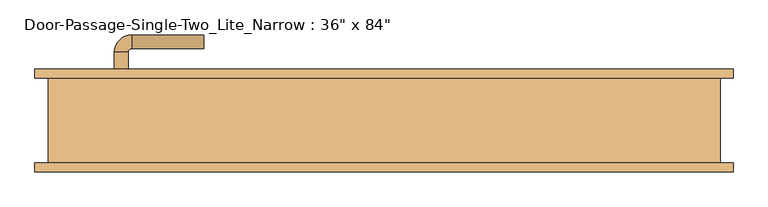
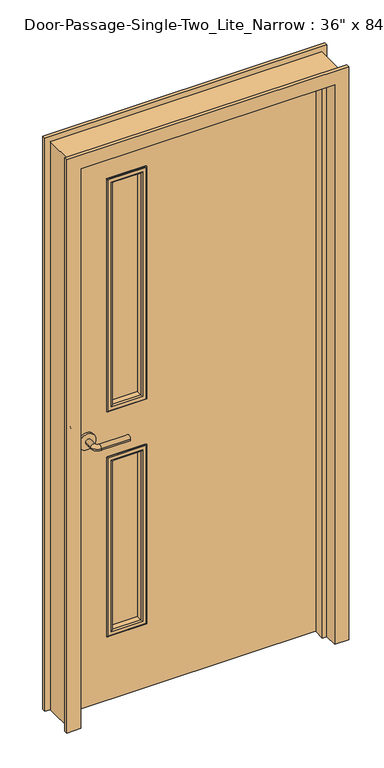
"""IFC4 building model written with IfcOpenShell, lengths in millimetres: door geometry."""

from ifc_helpers import new_model, si_unit, point, frame, frame_2d, origin, place, context, project, spatial, polyline, circle_curve, ellipse_curve, trimmed, segment, composite_curve, outline, extrude, faceted_brep, source, transform, mapped, element, save
from ifc_brep_helpers import plane_surface, cylinder_surface, revolved_surface, advanced_brep


def door_dba893c0(model_context):
    return source(origin(), model_context, "Body", "SolidModel", [
        advanced_brep(
        [(-392.190625, 15.8125, 1016.0), (-372.190625, 15.8125, 1016.0), (-372.190625, -14.1875, 1016.0), (-392.190625, -14.1875, 1016.0), (-367.190625, -19.1875, 1016.0), (-367.190625, -39.1875, 1016.0), (-262.190625, -39.1875, 1016.0), (-262.190625, -19.1875, 1016.0)],
        [
            (0, 1, circle_curve(frame((-382.190625, 15.8125, 1016.0), z_axis=(0.0, 1.0, 0.0), x_axis=(1.0, 0.0, 0.0)), 10.0)),
            (1, 0, circle_curve(frame((-382.190625, 15.8125, 1016.0), z_axis=(0.0, 1.0, 0.0), x_axis=(1.0, 0.0, 0.0)), 10.0)),
            (1, 2),
            (2, 3, circle_curve(frame((-382.190625, -14.1875, 1016.0), z_axis=(0.0, 1.0, 0.0), x_axis=(1.0, 0.0, 0.0)), 10.0)),
            (3, 0),
            (3, 2, circle_curve(frame((-382.190625, -14.1875, 1016.0), z_axis=(0.0, 1.0, 0.0), x_axis=(1.0, 0.0, 0.0)), 10.0)),
            (4, 5, circle_curve(frame((-367.190625, -29.1875, 1016.0), z_axis=(-1.0, 0.0, 0.0), x_axis=(0.0, 1.0, 0.0)), 10.0)),
            (5, 3, circle_curve(frame((-367.190625, -14.1875, 1016.0), z_axis=(0.0, 0.0, -1.0), x_axis=(-1.0, 0.0, 0.0)), 25.0)),
            (2, 4, circle_curve(frame((-367.190625, -14.1875, 1016.0), z_axis=(0.0, 0.0, 1.0), x_axis=(-1.0, 0.0, 0.0)), 5.0)),
            (5, 4, circle_curve(frame((-367.190625, -29.1875, 1016.0), z_axis=(-1.0, 0.0, 0.0), x_axis=(0.0, 1.0, 0.0)), 10.0)),
            (6, 7, circle_curve(frame((-262.190625, -29.1875, 1016.0), z_axis=(1.0, 0.0, 0.0), x_axis=(0.0, 1.0, 0.0)), 10.0)),
            (7, 6, circle_curve(frame((-262.190625, -29.1875, 1016.0), z_axis=(1.0, 0.0, 0.0), x_axis=(0.0, 1.0, 0.0)), 10.0)),
            (4, 7),
            (6, 5),
        ],
        [
            plane_surface(frame((-382.190625, 15.8125, 1016.0), z_axis=(0.0, 1.0, 0.0), x_axis=(0.0, 0.0, 1.0))),
            cylinder_surface(frame((-382.190625, 15.8125, 1016.0), z_axis=(0.0, 1.0, 0.0), x_axis=(1.0, 0.0, 0.0)), 10.0),
            revolved_surface(trimmed(ellipse_curve(frame((-382.190625, -14.1875, 1016.0), z_axis=(0.0, -1.0, 0.0), x_axis=(1.0, 0.0, 0.0)), 10.0, 10.0), [point((-392.190625, -14.1875, 1016.0))], [point((-372.190625, -14.1875, 1016.0))], True, "CARTESIAN"), (-367.190625, -14.1875, 1016.0), (0.0, 0.0, -1.0)),
            revolved_surface(trimmed(ellipse_curve(frame((-382.190625, -14.1875, 1016.0), z_axis=(0.0, -1.0, 0.0), x_axis=(1.0, 0.0, 0.0)), 10.0, 10.0), [point((-372.190625, -14.1875, 1016.0))], [point((-392.190625, -14.1875, 1016.0))], True, "CARTESIAN"), (-367.190625, -14.1875, 1016.0), (0.0, 0.0, -1.0)),
            plane_surface(frame((-262.190625, -29.1875, 1016.0), z_axis=(1.0, 0.0, 0.0), x_axis=(0.0, 0.0, 1.0))),
            cylinder_surface(frame((-367.190625, -29.1875, 1016.0), z_axis=(-1.0, 0.0, 0.0), x_axis=(0.0, 1.0, 0.0)), 10.0),
        ],
        [
            (0, [[1, 2]]),
            (1, [[3, 4, 5, -2]]),
            (1, [[-5, 6, -3, -1]]),
            (2, [[7, 8, -4, 9]]),
            (3, [[10, -9, -6, -8]]),
            (4, [[11, 12]]),
            (5, [[13, -11, 14, -7]]),
            (5, [[-14, -12, -13, -10]]),
        ],
    ),
        extrude(outline(composite_curve([segment(trimmed(circle_curve(frame_2d((1016.0, -384.690625)), 30.0), [point((1016.0, -414.690625))], [point((1016.0, -354.690625))], False, "CARTESIAN"), True, "CONTINUOUS"), segment(trimmed(circle_curve(frame_2d((1016.0, -384.690625)), 30.0), [point((1016.0, -354.690625))], [point((1016.0, -414.690625))], False, "CARTESIAN"), True, "CONTINUOUS")], self_intersect=False)), frame((0.0, 15.8125, 0.0), z_axis=(0.0, 1.0, 0.0), x_axis=(0.0, 0.0, 1.0)), (0.0, 0.0, 1.0), 8.0),
        advanced_brep(
        [(-392.190625, 76.2625, 1016.0), (-372.190625, 76.2625, 1016.0), (-392.190625, 106.2625, 1016.0), (-372.190625, 106.2625, 1016.0), (-367.190625, 111.2625, 1016.0), (-367.190625, 131.2625, 1016.0), (-262.190625, 131.2625, 1016.0), (-262.190625, 111.2625, 1016.0)],
        [
            (0, 1, circle_curve(frame((-382.190625, 76.2625, 1016.0), z_axis=(0.0, -1.0, 0.0), x_axis=(1.0, 0.0, 0.0)), 10.0)),
            (1, 0, circle_curve(frame((-382.190625, 76.2625, 1016.0), z_axis=(0.0, -1.0, 0.0), x_axis=(1.0, 0.0, 0.0)), 10.0)),
            (0, 2),
            (2, 3, circle_curve(frame((-382.190625, 106.2625, 1016.0), z_axis=(0.0, -1.0, 0.0), x_axis=(1.0, 0.0, 0.0)), 10.0)),
            (3, 1),
            (3, 2, circle_curve(frame((-382.190625, 106.2625, 1016.0), z_axis=(0.0, -1.0, 0.0), x_axis=(1.0, 0.0, 0.0)), 10.0)),
            (4, 3, circle_curve(frame((-367.190625, 106.2625, 1016.0), z_axis=(0.0, 0.0, 1.0), x_axis=(-1.0, 0.0, 0.0)), 5.0)),
            (2, 5, circle_curve(frame((-367.190625, 106.2625, 1016.0), z_axis=(0.0, 0.0, -1.0), x_axis=(-1.0, 0.0, 0.0)), 25.0)),
            (5, 4, circle_curve(frame((-367.190625, 121.2625, 1016.0), z_axis=(-1.0, 0.0, 0.0), x_axis=(0.0, -1.0, 0.0)), 10.0)),
            (4, 5, circle_curve(frame((-367.190625, 121.2625, 1016.0), z_axis=(-1.0, 0.0, 0.0), x_axis=(0.0, -1.0, 0.0)), 10.0)),
            (6, 7, circle_curve(frame((-262.190625, 121.2625, 1016.0), z_axis=(1.0, 0.0, 0.0), x_axis=(0.0, -1.0, 0.0)), 10.0)),
            (7, 6, circle_curve(frame((-262.190625, 121.2625, 1016.0), z_axis=(1.0, 0.0, 0.0), x_axis=(0.0, -1.0, 0.0)), 10.0)),
            (5, 6),
            (7, 4),
        ],
        [
            plane_surface(frame((-382.190625, 76.2625, 1016.0), z_axis=(0.0, -1.0, 0.0), x_axis=(0.0, 0.0, 1.0))),
            cylinder_surface(frame((-382.190625, 76.2625, 1016.0), z_axis=(0.0, -1.0, 0.0), x_axis=(1.0, 0.0, 0.0)), 10.0),
            revolved_surface(trimmed(ellipse_curve(frame((-382.190625, 106.2625, 1016.0), z_axis=(0.0, -1.0, 0.0), x_axis=(1.0, 0.0, 0.0)), 10.0, 10.0), [point((-392.190625, 106.2625, 1016.0))], [point((-372.190625, 106.2625, 1016.0))], True, "CARTESIAN"), (-367.190625, 106.2625, 1016.0), (0.0, 0.0, -1.0)),
            revolved_surface(trimmed(ellipse_curve(frame((-382.190625, 106.2625, 1016.0), z_axis=(0.0, -1.0, 0.0), x_axis=(1.0, 0.0, 0.0)), 10.0, 10.0), [point((-372.190625, 106.2625, 1016.0))], [point((-392.190625, 106.2625, 1016.0))], True, "CARTESIAN"), (-367.190625, 106.2625, 1016.0), (0.0, 0.0, -1.0)),
            plane_surface(frame((-262.190625, 121.2625, 1016.0), z_axis=(1.0, 0.0, 0.0), x_axis=(0.0, 0.0, 1.0))),
            cylinder_surface(frame((-367.190625, 121.2625, 1016.0), z_axis=(-1.0, 0.0, 0.0), x_axis=(0.0, -1.0, 0.0)), 10.0),
        ],
        [
            (0, [[1, 2]]),
            (1, [[-1, 3, 4, 5]]),
            (1, [[-2, -5, 6, -3]]),
            (2, [[7, -4, 8, 9]]),
            (3, [[-8, -6, -7, 10]]),
            (4, [[11, 12]]),
            (5, [[-9, 13, -12, 14]]),
            (5, [[-10, -14, -11, -13]]),
        ],
    ),
        extrude(outline(composite_curve([segment(trimmed(circle_curve(frame_2d((1016.0, -384.690625)), 30.0), [point((1016.0, -414.690625))], [point((1016.0, -354.690625))], False, "CARTESIAN"), True, "CONTINUOUS"), segment(trimmed(circle_curve(frame_2d((1016.0, -384.690625)), 30.0), [point((1016.0, -354.690625))], [point((1016.0, -414.690625))], False, "CARTESIAN"), True, "CONTINUOUS")], self_intersect=False)), frame((0.0, 68.2625, 0.0), z_axis=(0.0, 1.0, 0.0), x_axis=(0.0, 0.0, 1.0)), (0.0, 0.0, 1.0), 8.0),
        faceted_brep([(457.2, 80.9625, 0.0), (508.0, 80.9625, 0.0), (508.0, 68.2625, 0.0), (488.95, 68.2625, 0.0), (488.95, -55.5625, 0.0), (508.0, -55.5625, 0.0), (508.0, -68.2625, 0.0), (457.2, -68.2625, 0.0), (457.2, -19.05, 0.0), (441.325, -19.05, 0.0), (441.325, 19.05, 0.0), (457.2, 19.05, 0.0), (457.2, 80.9625, 2133.6), (-457.2, 80.9625, 2133.6), (-457.2, 80.9625, 0.0), (-508.0, 80.9625, 0.0), (-508.0, 80.9625, 2184.4), (508.0, 80.9625, 2184.4), (508.0, 68.2625, 2184.4), (-508.0, 68.2625, 2184.4), (-508.0, 68.2625, 0.0), (-488.95, 68.2625, 0.0), (-488.95, 68.2625, 2165.35), (488.95, 68.2625, 2165.35), (488.95, -55.5625, 2165.35), (-488.95, -55.5625, 2165.35), (-488.95, -55.5625, 0.0), (-508.0, -55.5625, 0.0), (-508.0, -55.5625, 2184.4), (508.0, -55.5625, 2184.4), (508.0, -68.2625, 2184.4), (-508.0, -68.2625, 2184.4), (-508.0, -68.2625, 0.0), (-457.2, -68.2625, 0.0), (-457.2, -68.2625, 2133.6), (457.2, -68.2625, 2133.6), (457.2, -19.05, 2133.6), (-457.2, -19.05, 2133.6), (-457.2, -19.05, 0.0), (-441.325, -19.05, 0.0), (-441.325, -19.05, 2117.725), (441.325, -19.05, 2117.725), (441.325, 19.05, 2117.725), (-441.325, 19.05, 2117.725), (-441.325, 19.05, 0.0), (-457.2, 19.05, 0.0), (-457.2, 19.05, 2133.6), (457.2, 19.05, 2133.6)], [[[0, 1, 2, 3, 4, 5, 6, 7, 8, 9, 10, 11]], [[1, 0, 12, 13, 14, 15, 16, 17]], [[2, 1, 17, 18]], [[3, 2, 18, 19, 20, 21, 22, 23]], [[4, 3, 23, 24]], [[5, 4, 24, 25, 26, 27, 28, 29]], [[6, 5, 29, 30]], [[7, 6, 30, 31, 32, 33, 34, 35]], [[8, 7, 35, 36]], [[9, 8, 36, 37, 38, 39, 40, 41]], [[10, 9, 41, 42]], [[11, 10, 42, 43, 44, 45, 46, 47]], [[0, 11, 47, 12]], [[18, 17, 16, 19]], [[24, 23, 22, 25]], [[30, 29, 28, 31]], [[36, 35, 34, 37]], [[42, 41, 40, 43]], [[12, 47, 46, 13]], [[14, 45, 44, 39, 38, 33, 32, 27, 26, 21, 20, 15]], [[19, 16, 15, 20]], [[25, 22, 21, 26]], [[31, 28, 27, 32]], [[37, 34, 33, 38]], [[43, 40, 39, 44]], [[13, 46, 45, 14]]]),
        extrude(outline(polyline([(2133.6, -457.2), (0.0, -457.2), (0.0, 457.2), (2133.6, 457.2), (2133.6, -457.2)]), holes=[polyline([(1981.2, -304.8), (1981.2, -177.8), (1111.25, -177.8), (1111.25, -304.8), (1981.2, -304.8)]), polyline([(920.75, -304.8), (920.75, -177.8), (254.0, -177.8), (254.0, -304.8), (920.75, -304.8)])]), frame((0.0, 23.8125, 0.0), z_axis=(0.0, 1.0, 0.0), x_axis=(0.0, 0.0, 1.0)), (0.0, 0.0, 1.0), 44.45),
        extrude(outline(polyline([(-177.8, 42.8625), (-304.8, 42.8625), (-304.8, 49.2125), (-177.8, 49.2125), (-177.8, 42.8625)])), frame((0.0, 0.0, 1111.25), z_axis=(0.0, 0.0, 1.0), x_axis=(1.0, 0.0, 0.0)), (0.0, 0.0, 1.0), 869.95),
        extrude(outline(polyline([(-177.8, 42.8625), (-304.8, 42.8625), (-304.8, 49.2125), (-177.8, 49.2125), (-177.8, 42.8625)])), frame((0.0, 0.0, 254.0), z_axis=(0.0, 0.0, 1.0), x_axis=(1.0, 0.0, 0.0)), (0.0, 0.0, 1.0), 666.75),
        advanced_brep(
        [(-177.8, 42.8625, 920.75), (-177.8, 23.8125, 920.75), (-177.8, 23.8125, 254.0), (-177.8, 42.8625, 254.0), (-189.8, 22.8125, 908.75), (-189.8, 42.8625, 908.75), (-189.8, 42.8625, 266.0), (-189.8, 22.8125, 266.0), (-184.8, 17.8125, 913.75), (-184.8, 17.8125, 261.0), (-169.8, 19.8125, 928.75), (-171.8, 17.8125, 926.75), (-171.8, 17.8125, 248.0), (-169.8, 19.8125, 246.0), (-169.8, 23.8125, 928.75), (-169.8, 23.8125, 246.0), (-304.8, 23.8125, 254.0), (-304.8, 42.8625, 254.0), (-292.8, 42.8625, 266.0), (-292.8, 22.8125, 266.0), (-297.8, 17.8125, 261.0), (-310.8, 17.8125, 248.0), (-312.8, 19.8125, 246.0), (-312.8, 23.8125, 246.0), (-304.8, 23.8125, 920.75), (-304.8, 42.8625, 920.75), (-292.8, 42.8625, 908.75), (-292.8, 22.8125, 908.75), (-297.8, 17.8125, 913.75), (-310.8, 17.8125, 926.75), (-312.8, 19.8125, 928.75), (-312.8, 23.8125, 928.75)],
        [
            (0, 1),
            (1, 2),
            (2, 3),
            (3, 0),
            (4, 5),
            (5, 6),
            (6, 7),
            (7, 4),
            (8, 4, ellipse_curve(frame((-184.8, 22.8125, 913.75), z_axis=(0.7071067811865475, 0.0, -0.7071067811865475), x_axis=(0.7071067811865474, 0.0, 0.7071067811865476)), 7.0710678, 5.0)),
            (7, 9, ellipse_curve(frame((-184.8, 22.8125, 261.0), z_axis=(0.7071067811865475, 0.0, 0.7071067811865475), x_axis=(-0.7071067811865474, 0.0, 0.7071067811865476)), 7.0710678, 5.0)),
            (9, 8),
            (10, 11, ellipse_curve(frame((-171.8, 19.8125, 926.75), z_axis=(0.7071067811865475, 0.0, -0.7071067811865475), x_axis=(0.7071067811865474, 0.0, 0.7071067811865476)), 2.8284271, 2.0)),
            (11, 12),
            (12, 13, ellipse_curve(frame((-171.8, 19.8125, 248.0), z_axis=(0.7071067811865475, 0.0, 0.7071067811865475), x_axis=(-0.7071067811865474, 0.0, 0.7071067811865476)), 2.8284271, 2.0)),
            (13, 10),
            (14, 10),
            (13, 15),
            (15, 14),
            (2, 16),
            (16, 17),
            (17, 3),
            (6, 18),
            (18, 19),
            (19, 7),
            (19, 20, ellipse_curve(frame((-297.8, 22.8125, 261.0), z_axis=(0.7071067811865475, 0.0, -0.7071067811865475), x_axis=(0.7071067811865476, 0.0, 0.7071067811865474)), 7.0710678, 5.0)),
            (20, 9),
            (12, 21),
            (21, 22, ellipse_curve(frame((-310.8, 19.8125, 248.0), z_axis=(0.7071067811865475, 0.0, -0.7071067811865475), x_axis=(0.7071067811865476, 0.0, 0.7071067811865474)), 2.8284271, 2.0)),
            (22, 13),
            (22, 23),
            (23, 15),
            (16, 24),
            (24, 25),
            (25, 17),
            (18, 26),
            (26, 27),
            (27, 19),
            (27, 28, ellipse_curve(frame((-297.8, 22.8125, 913.75), z_axis=(-0.7071067811865475, 0.0, -0.7071067811865475), x_axis=(0.7071067811865474, 0.0, -0.7071067811865476)), 7.0710678, 5.0)),
            (28, 20),
            (21, 29),
            (29, 30, ellipse_curve(frame((-310.8, 19.8125, 926.75), z_axis=(-0.7071067811865475, 0.0, -0.7071067811865475), x_axis=(0.7071067811865474, 0.0, -0.7071067811865476)), 2.8284271, 2.0)),
            (30, 22),
            (30, 31),
            (31, 23),
            (31, 14),
            (1, 24),
            (0, 25),
            (5, 26),
            (4, 27),
            (8, 28),
            (11, 29),
            (10, 30),
        ],
        [
            plane_surface(frame((-177.8, 23.8125, 920.75), z_axis=(1.0, 0.0, 0.0), x_axis=(0.0, 0.0, -1.0))),
            plane_surface(frame((-189.8, 42.8625, 908.75), z_axis=(-1.0, 0.0, 0.0), x_axis=(0.0, 0.0, -1.0))),
            cylinder_surface(frame((-184.8, 22.8125, 920.75), z_axis=(0.0, 0.0, 1.0), x_axis=(1.0, 0.0, 0.0)), 5.0),
            cylinder_surface(frame((-171.8, 19.8125, 920.75), z_axis=(0.0, 0.0, 1.0), x_axis=(1.0, 0.0, 0.0)), 2.0),
            plane_surface(frame((-169.8, 19.8125, 928.75), z_axis=(1.0, 0.0, 0.0), x_axis=(0.0, 0.0, -1.0))),
            plane_surface(frame((-177.8, 23.8125, 254.0), z_axis=(0.0, 0.0, -1.0), x_axis=(-1.0, 0.0, 0.0))),
            plane_surface(frame((-189.8, 42.8625, 266.0), z_axis=(0.0, 0.0, 1.0), x_axis=(-1.0, 0.0, 0.0))),
            cylinder_surface(frame((-177.8, 22.8125, 261.0), z_axis=(1.0, 0.0, 0.0), x_axis=(0.0, 0.0, -1.0)), 5.0),
            cylinder_surface(frame((-177.8, 19.8125, 248.0), z_axis=(1.0, 0.0, 0.0), x_axis=(0.0, 0.0, -1.0)), 2.0),
            plane_surface(frame((-169.8, 19.8125, 246.0), z_axis=(0.0, 0.0, -1.0), x_axis=(-1.0, 0.0, 0.0))),
            plane_surface(frame((-304.8, 23.8125, 254.0), z_axis=(-1.0, 0.0, 0.0), x_axis=(0.0, 0.0, 1.0))),
            plane_surface(frame((-292.8, 42.8625, 266.0), z_axis=(1.0, 0.0, 0.0), x_axis=(0.0, 0.0, 1.0))),
            cylinder_surface(frame((-297.8, 22.8125, 254.0), z_axis=(0.0, 0.0, -1.0), x_axis=(-1.0, 0.0, 0.0)), 5.0),
            cylinder_surface(frame((-310.8, 19.8125, 254.0), z_axis=(0.0, 0.0, -1.0), x_axis=(-1.0, 0.0, 0.0)), 2.0),
            plane_surface(frame((-312.8, 19.8125, 246.0), z_axis=(-1.0, 0.0, 0.0), x_axis=(0.0, 0.0, 1.0))),
            plane_surface(frame((-312.8, 23.8125, 928.75), z_axis=(0.0, 1.0, 0.0), x_axis=(1.0, 0.0, 0.0))),
            plane_surface(frame((-304.8, 23.8125, 920.75), z_axis=(0.0, 0.0, 1.0), x_axis=(1.0, 0.0, 0.0))),
            plane_surface(frame((-304.8, 42.8625, 920.75), z_axis=(0.0, 1.0, 0.0), x_axis=(1.0, 0.0, 0.0))),
            plane_surface(frame((-292.8, 42.8625, 908.75), z_axis=(0.0, 0.0, -1.0), x_axis=(1.0, 0.0, 0.0))),
            cylinder_surface(frame((-304.8, 22.8125, 913.75), z_axis=(-1.0, 0.0, 0.0), x_axis=(0.0, 0.0, 1.0)), 5.0),
            plane_surface(frame((-297.8, 17.8125, 913.75), z_axis=(0.0, -1.0, 0.0), x_axis=(1.0, 0.0, 0.0))),
            cylinder_surface(frame((-304.8, 19.8125, 926.75), z_axis=(-1.0, 0.0, 0.0), x_axis=(0.0, 0.0, 1.0)), 2.0),
            plane_surface(frame((-312.8, 19.8125, 928.75), z_axis=(0.0, 0.0, 1.0), x_axis=(1.0, 0.0, 0.0))),
        ],
        [
            (0, [[1, 2, 3, 4]]),
            (1, [[5, 6, 7, 8]]),
            (2, [[9, -8, 10, 11]]),
            (3, [[12, 13, 14, 15]]),
            (4, [[16, -15, 17, 18]]),
            (5, [[-3, 19, 20, 21]]),
            (6, [[-7, 22, 23, 24]]),
            (7, [[-10, -24, 25, 26]]),
            (8, [[-14, 27, 28, 29]]),
            (9, [[-17, -29, 30, 31]]),
            (10, [[-20, 32, 33, 34]]),
            (11, [[-23, 35, 36, 37]]),
            (12, [[-25, -37, 38, 39]]),
            (13, [[-28, 40, 41, 42]]),
            (14, [[-30, -42, 43, 44]]),
            (15, [[-31, -44, 45, -18], [46, -32, -19, -2]]),
            (16, [[-33, -46, -1, 47]]),
            (17, [[-21, -34, -47, -4], [48, -35, -22, -6]]),
            (18, [[-36, -48, -5, 49]]),
            (19, [[-38, -49, -9, 50]]),
            (20, [[51, -40, -27, -13], [-26, -39, -50, -11]]),
            (21, [[-41, -51, -12, 52]]),
            (22, [[-43, -52, -16, -45]]),
        ],
    ),
        advanced_brep(
        [(-304.8, 49.2125, 920.75), (-304.8, 68.2625, 920.75), (-304.8, 68.2625, 254.0), (-304.8, 49.2125, 254.0), (-292.8, 69.2625, 908.75), (-292.8, 49.2125, 908.75), (-292.8, 49.2125, 266.0), (-292.8, 69.2625, 266.0), (-297.8, 74.2625, 913.75), (-297.8, 74.2625, 261.0), (-312.8, 72.2625, 928.75), (-310.8, 74.2625, 926.75), (-310.8, 74.2625, 248.0), (-312.8, 72.2625, 246.0), (-312.8, 68.2625, 928.75), (-312.8, 68.2625, 246.0), (-177.8, 68.2625, 254.0), (-177.8, 49.2125, 254.0), (-189.8, 49.2125, 266.0), (-189.8, 69.2625, 266.0), (-184.8, 74.2625, 261.0), (-171.8, 74.2625, 248.0), (-169.8, 72.2625, 246.0), (-169.8, 68.2625, 246.0), (-177.8, 68.2625, 920.75), (-177.8, 49.2125, 920.75), (-189.8, 49.2125, 908.75), (-189.8, 69.2625, 908.75), (-184.8, 74.2625, 913.75), (-171.8, 74.2625, 926.75), (-169.8, 72.2625, 928.75), (-169.8, 68.2625, 928.75)],
        [
            (0, 1),
            (1, 2),
            (2, 3),
            (3, 0),
            (4, 5),
            (5, 6),
            (6, 7),
            (7, 4),
            (8, 4, ellipse_curve(frame((-297.8, 69.2625, 913.75), z_axis=(-0.7071067811865475, 0.0, -0.7071067811865475), x_axis=(-0.7071067811865474, 0.0, 0.7071067811865476)), 7.0710678, 5.0)),
            (7, 9, ellipse_curve(frame((-297.8, 69.2625, 261.0), z_axis=(-0.7071067811865475, 0.0, 0.7071067811865475), x_axis=(0.7071067811865474, 0.0, 0.7071067811865476)), 7.0710678, 5.0)),
            (9, 8),
            (10, 11, ellipse_curve(frame((-310.8, 72.2625, 926.75), z_axis=(-0.7071067811865475, 0.0, -0.7071067811865475), x_axis=(-0.7071067811865474, 0.0, 0.7071067811865476)), 2.8284271, 2.0)),
            (11, 12),
            (12, 13, ellipse_curve(frame((-310.8, 72.2625, 248.0), z_axis=(-0.7071067811865475, 0.0, 0.7071067811865475), x_axis=(0.7071067811865474, 0.0, 0.7071067811865476)), 2.8284271, 2.0)),
            (13, 10),
            (14, 10),
            (13, 15),
            (15, 14),
            (2, 16),
            (16, 17),
            (17, 3),
            (6, 18),
            (18, 19),
            (19, 7),
            (19, 20, ellipse_curve(frame((-184.8, 69.2625, 261.0), z_axis=(-0.7071067811865475, 0.0, -0.7071067811865475), x_axis=(-0.7071067811865476, 0.0, 0.7071067811865474)), 7.0710678, 5.0)),
            (20, 9),
            (12, 21),
            (21, 22, ellipse_curve(frame((-171.8, 72.2625, 248.0), z_axis=(-0.7071067811865475, 0.0, -0.7071067811865475), x_axis=(-0.7071067811865476, 0.0, 0.7071067811865474)), 2.8284271, 2.0)),
            (22, 13),
            (22, 23),
            (23, 15),
            (16, 24),
            (24, 25),
            (25, 17),
            (18, 26),
            (26, 27),
            (27, 19),
            (27, 28, ellipse_curve(frame((-184.8, 69.2625, 913.75), z_axis=(0.7071067811865475, 0.0, -0.7071067811865475), x_axis=(-0.7071067811865474, 0.0, -0.7071067811865476)), 7.0710678, 5.0)),
            (28, 20),
            (21, 29),
            (29, 30, ellipse_curve(frame((-171.8, 72.2625, 926.75), z_axis=(0.7071067811865475, 0.0, -0.7071067811865475), x_axis=(-0.7071067811865474, 0.0, -0.7071067811865476)), 2.8284271, 2.0)),
            (30, 22),
            (30, 31),
            (31, 23),
            (31, 14),
            (1, 24),
            (0, 25),
            (5, 26),
            (4, 27),
            (8, 28),
            (11, 29),
            (10, 30),
        ],
        [
            plane_surface(frame((-304.8, 68.2625, 920.75), z_axis=(-1.0, 0.0, 0.0), x_axis=(0.0, 0.0, -1.0))),
            plane_surface(frame((-292.8, 49.2125, 908.75), z_axis=(1.0, 0.0, 0.0), x_axis=(0.0, 0.0, -1.0))),
            cylinder_surface(frame((-297.8, 69.2625, 920.75), z_axis=(0.0, 0.0, 1.0), x_axis=(-1.0, 0.0, 0.0)), 5.0),
            cylinder_surface(frame((-310.8, 72.2625, 920.75), z_axis=(0.0, 0.0, 1.0), x_axis=(-1.0, 0.0, 0.0)), 2.0),
            plane_surface(frame((-312.8, 72.2625, 928.75), z_axis=(-1.0, 0.0, 0.0), x_axis=(0.0, 0.0, -1.0))),
            plane_surface(frame((-304.8, 68.2625, 254.0), z_axis=(0.0, 0.0, -1.0), x_axis=(1.0, 0.0, 0.0))),
            plane_surface(frame((-292.8, 49.2125, 266.0), z_axis=(0.0, 0.0, 1.0), x_axis=(1.0, 0.0, 0.0))),
            cylinder_surface(frame((-304.8, 69.2625, 261.0), z_axis=(-1.0, 0.0, 0.0), x_axis=(0.0, 0.0, -1.0)), 5.0),
            cylinder_surface(frame((-304.8, 72.2625, 248.0), z_axis=(-1.0, 0.0, 0.0), x_axis=(0.0, 0.0, -1.0)), 2.0),
            plane_surface(frame((-312.8, 72.2625, 246.0), z_axis=(0.0, 0.0, -1.0), x_axis=(1.0, 0.0, 0.0))),
            plane_surface(frame((-177.8, 68.2625, 254.0), z_axis=(1.0, 0.0, 0.0), x_axis=(0.0, 0.0, 1.0))),
            plane_surface(frame((-189.8, 49.2125, 266.0), z_axis=(-1.0, 0.0, 0.0), x_axis=(0.0, 0.0, 1.0))),
            cylinder_surface(frame((-184.8, 69.2625, 254.0), z_axis=(0.0, 0.0, -1.0), x_axis=(1.0, 0.0, 0.0)), 5.0),
            cylinder_surface(frame((-171.8, 72.2625, 254.0), z_axis=(0.0, 0.0, -1.0), x_axis=(1.0, 0.0, 0.0)), 2.0),
            plane_surface(frame((-169.8, 72.2625, 246.0), z_axis=(1.0, 0.0, 0.0), x_axis=(0.0, 0.0, 1.0))),
            plane_surface(frame((-169.8, 68.2625, 928.75), z_axis=(0.0, -1.0, 0.0), x_axis=(-1.0, 0.0, 0.0))),
            plane_surface(frame((-177.8, 68.2625, 920.75), z_axis=(0.0, 0.0, 1.0), x_axis=(-1.0, 0.0, 0.0))),
            plane_surface(frame((-177.8, 49.2125, 920.75), z_axis=(0.0, -1.0, 0.0), x_axis=(-1.0, 0.0, 0.0))),
            plane_surface(frame((-189.8, 49.2125, 908.75), z_axis=(0.0, 0.0, -1.0), x_axis=(-1.0, 0.0, 0.0))),
            cylinder_surface(frame((-177.8, 69.2625, 913.75), z_axis=(1.0, 0.0, 0.0), x_axis=(0.0, 0.0, 1.0)), 5.0),
            plane_surface(frame((-184.8, 74.2625, 913.75), z_axis=(0.0, 1.0, 0.0), x_axis=(-1.0, 0.0, 0.0))),
            cylinder_surface(frame((-177.8, 72.2625, 926.75), z_axis=(1.0, 0.0, 0.0), x_axis=(0.0, 0.0, 1.0)), 2.0),
            plane_surface(frame((-169.8, 72.2625, 928.75), z_axis=(0.0, 0.0, 1.0), x_axis=(-1.0, 0.0, 0.0))),
        ],
        [
            (0, [[1, 2, 3, 4]]),
            (1, [[5, 6, 7, 8]]),
            (2, [[9, -8, 10, 11]]),
            (3, [[12, 13, 14, 15]]),
            (4, [[16, -15, 17, 18]]),
            (5, [[-3, 19, 20, 21]]),
            (6, [[-7, 22, 23, 24]]),
            (7, [[-10, -24, 25, 26]]),
            (8, [[-14, 27, 28, 29]]),
            (9, [[-17, -29, 30, 31]]),
            (10, [[-20, 32, 33, 34]]),
            (11, [[-23, 35, 36, 37]]),
            (12, [[-25, -37, 38, 39]]),
            (13, [[-28, 40, 41, 42]]),
            (14, [[-30, -42, 43, 44]]),
            (15, [[-31, -44, 45, -18], [46, -32, -19, -2]]),
            (16, [[-33, -46, -1, 47]]),
            (17, [[-21, -34, -47, -4], [48, -35, -22, -6]]),
            (18, [[-36, -48, -5, 49]]),
            (19, [[-38, -49, -9, 50]]),
            (20, [[51, -40, -27, -13], [-26, -39, -50, -11]]),
            (21, [[-41, -51, -12, 52]]),
            (22, [[-43, -52, -16, -45]]),
        ],
    ),
        advanced_brep(
        [(-304.8, 42.8625, 1111.25), (-304.8, 23.8125, 1111.25), (-304.8, 23.8125, 1981.2), (-304.8, 42.8625, 1981.2), (-292.8, 22.8125, 1123.25), (-292.8, 42.8625, 1123.25), (-292.8, 42.8625, 1969.2), (-292.8, 22.8125, 1969.2), (-297.8, 17.8125, 1118.25), (-297.8, 17.8125, 1974.2), (-312.8, 19.8125, 1103.25), (-310.8, 17.8125, 1105.25), (-310.8, 17.8125, 1987.2), (-312.8, 19.8125, 1989.2), (-312.8, 23.8125, 1103.25), (-312.8, 23.8125, 1989.2), (-177.8, 23.8125, 1981.2), (-177.8, 42.8625, 1981.2), (-189.8, 42.8625, 1969.2), (-189.8, 22.8125, 1969.2), (-184.8, 17.8125, 1974.2), (-171.8, 17.8125, 1987.2), (-169.8, 19.8125, 1989.2), (-169.8, 23.8125, 1989.2), (-177.8, 23.8125, 1111.25), (-177.8, 42.8625, 1111.25), (-189.8, 42.8625, 1123.25), (-189.8, 22.8125, 1123.25), (-184.8, 17.8125, 1118.25), (-171.8, 17.8125, 1105.25), (-169.8, 19.8125, 1103.25), (-169.8, 23.8125, 1103.25)],
        [
            (0, 1),
            (1, 2),
            (2, 3),
            (3, 0),
            (4, 5),
            (5, 6),
            (6, 7),
            (7, 4),
            (8, 4, ellipse_curve(frame((-297.8, 22.8125, 1118.25), z_axis=(-0.7071067811865475, 0.0, 0.7071067811865475), x_axis=(-0.7071067811865474, 0.0, -0.7071067811865476)), 7.0710678, 5.0)),
            (7, 9, ellipse_curve(frame((-297.8, 22.8125, 1974.2), z_axis=(-0.7071067811865475, 0.0, -0.7071067811865475), x_axis=(0.7071067811865474, 0.0, -0.7071067811865476)), 7.0710678, 5.0)),
            (9, 8),
            (10, 11, ellipse_curve(frame((-310.8, 19.8125, 1105.25), z_axis=(-0.7071067811865475, 0.0, 0.7071067811865475), x_axis=(-0.7071067811865474, 0.0, -0.7071067811865476)), 2.8284271, 2.0)),
            (11, 12),
            (12, 13, ellipse_curve(frame((-310.8, 19.8125, 1987.2), z_axis=(-0.7071067811865475, 0.0, -0.7071067811865475), x_axis=(0.7071067811865474, 0.0, -0.7071067811865476)), 2.8284271, 2.0)),
            (13, 10),
            (14, 10),
            (13, 15),
            (15, 14),
            (2, 16),
            (16, 17),
            (17, 3),
            (6, 18),
            (18, 19),
            (19, 7),
            (19, 20, ellipse_curve(frame((-184.8, 22.8125, 1974.2), z_axis=(-0.7071067811865475, 0.0, 0.7071067811865475), x_axis=(-0.7071067811865476, 0.0, -0.7071067811865474)), 7.0710678, 5.0)),
            (20, 9),
            (12, 21),
            (21, 22, ellipse_curve(frame((-171.8, 19.8125, 1987.2), z_axis=(-0.7071067811865475, 0.0, 0.7071067811865475), x_axis=(-0.7071067811865476, 0.0, -0.7071067811865474)), 2.8284271, 2.0)),
            (22, 13),
            (22, 23),
            (23, 15),
            (16, 24),
            (24, 25),
            (25, 17),
            (18, 26),
            (26, 27),
            (27, 19),
            (27, 28, ellipse_curve(frame((-184.8, 22.8125, 1118.25), z_axis=(0.7071067811865475, 0.0, 0.7071067811865475), x_axis=(-0.7071067811865474, 0.0, 0.7071067811865476)), 7.0710678, 5.0)),
            (28, 20),
            (21, 29),
            (29, 30, ellipse_curve(frame((-171.8, 19.8125, 1105.25), z_axis=(0.7071067811865475, 0.0, 0.7071067811865475), x_axis=(-0.7071067811865474, 0.0, 0.7071067811865476)), 2.8284271, 2.0)),
            (30, 22),
            (30, 31),
            (31, 23),
            (31, 14),
            (1, 24),
            (0, 25),
            (5, 26),
            (4, 27),
            (8, 28),
            (11, 29),
            (10, 30),
        ],
        [
            plane_surface(frame((-304.8, 23.8125, 1111.25), z_axis=(-1.0, 0.0, 0.0), x_axis=(0.0, 0.0, 1.0))),
            plane_surface(frame((-292.8, 42.8625, 1123.25), z_axis=(1.0, 0.0, 0.0), x_axis=(0.0, 0.0, 1.0))),
            cylinder_surface(frame((-297.8, 22.8125, 1111.25), z_axis=(0.0, 0.0, -1.0), x_axis=(-1.0, 0.0, 0.0)), 5.0),
            cylinder_surface(frame((-310.8, 19.8125, 1111.25), z_axis=(0.0, 0.0, -1.0), x_axis=(-1.0, 0.0, 0.0)), 2.0),
            plane_surface(frame((-312.8, 19.8125, 1103.25), z_axis=(-1.0, 0.0, 0.0), x_axis=(0.0, 0.0, 1.0))),
            plane_surface(frame((-304.8, 23.8125, 1981.2), z_axis=(0.0, 0.0, 1.0), x_axis=(1.0, 0.0, 0.0))),
            plane_surface(frame((-292.8, 42.8625, 1969.2), z_axis=(0.0, 0.0, -1.0), x_axis=(1.0, 0.0, 0.0))),
            cylinder_surface(frame((-304.8, 22.8125, 1974.2), z_axis=(-1.0, 0.0, 0.0), x_axis=(0.0, 0.0, 1.0)), 5.0),
            cylinder_surface(frame((-304.8, 19.8125, 1987.2), z_axis=(-1.0, 0.0, 0.0), x_axis=(0.0, 0.0, 1.0)), 2.0),
            plane_surface(frame((-312.8, 19.8125, 1989.2), z_axis=(0.0, 0.0, 1.0), x_axis=(1.0, 0.0, 0.0))),
            plane_surface(frame((-177.8, 23.8125, 1981.2), z_axis=(1.0, 0.0, 0.0), x_axis=(0.0, 0.0, -1.0))),
            plane_surface(frame((-189.8, 42.8625, 1969.2), z_axis=(-1.0, 0.0, 0.0), x_axis=(0.0, 0.0, -1.0))),
            cylinder_surface(frame((-184.8, 22.8125, 1981.2), z_axis=(0.0, 0.0, 1.0), x_axis=(1.0, 0.0, 0.0)), 5.0),
            cylinder_surface(frame((-171.8, 19.8125, 1981.2), z_axis=(0.0, 0.0, 1.0), x_axis=(1.0, 0.0, 0.0)), 2.0),
            plane_surface(frame((-169.8, 19.8125, 1989.2), z_axis=(1.0, 0.0, 0.0), x_axis=(0.0, 0.0, -1.0))),
            plane_surface(frame((-169.8, 23.8125, 1103.25), z_axis=(0.0, 1.0, 0.0), x_axis=(-1.0, 0.0, 0.0))),
            plane_surface(frame((-177.8, 23.8125, 1111.25), z_axis=(0.0, 0.0, -1.0), x_axis=(-1.0, 0.0, 0.0))),
            plane_surface(frame((-177.8, 42.8625, 1111.25), z_axis=(0.0, 1.0, 0.0), x_axis=(-1.0, 0.0, 0.0))),
            plane_surface(frame((-189.8, 42.8625, 1123.25), z_axis=(0.0, 0.0, 1.0), x_axis=(-1.0, 0.0, 0.0))),
            cylinder_surface(frame((-177.8, 22.8125, 1118.25), z_axis=(1.0, 0.0, 0.0), x_axis=(0.0, 0.0, -1.0)), 5.0),
            plane_surface(frame((-184.8, 17.8125, 1118.25), z_axis=(0.0, -1.0, 0.0), x_axis=(-1.0, 0.0, 0.0))),
            cylinder_surface(frame((-177.8, 19.8125, 1105.25), z_axis=(1.0, 0.0, 0.0), x_axis=(0.0, 0.0, -1.0)), 2.0),
            plane_surface(frame((-169.8, 19.8125, 1103.25), z_axis=(0.0, 0.0, -1.0), x_axis=(-1.0, 0.0, 0.0))),
        ],
        [
            (0, [[1, 2, 3, 4]]),
            (1, [[5, 6, 7, 8]]),
            (2, [[9, -8, 10, 11]]),
            (3, [[12, 13, 14, 15]]),
            (4, [[16, -15, 17, 18]]),
            (5, [[-3, 19, 20, 21]]),
            (6, [[-7, 22, 23, 24]]),
            (7, [[-10, -24, 25, 26]]),
            (8, [[-14, 27, 28, 29]]),
            (9, [[-17, -29, 30, 31]]),
            (10, [[-20, 32, 33, 34]]),
            (11, [[-23, 35, 36, 37]]),
            (12, [[-25, -37, 38, 39]]),
            (13, [[-28, 40, 41, 42]]),
            (14, [[-30, -42, 43, 44]]),
            (15, [[-31, -44, 45, -18], [46, -32, -19, -2]]),
            (16, [[-33, -46, -1, 47]]),
            (17, [[-21, -34, -47, -4], [48, -35, -22, -6]]),
            (18, [[-36, -48, -5, 49]]),
            (19, [[-38, -49, -9, 50]]),
            (20, [[51, -40, -27, -13], [-26, -39, -50, -11]]),
            (21, [[-41, -51, -12, 52]]),
            (22, [[-43, -52, -16, -45]]),
        ],
    ),
        advanced_brep(
        [(-304.8, 49.2125, 1981.2), (-304.8, 68.2625, 1981.2), (-304.8, 68.2625, 1111.25), (-304.8, 49.2125, 1111.25), (-292.8, 69.2625, 1969.2), (-292.8, 49.2125, 1969.2), (-292.8, 49.2125, 1123.25), (-292.8, 69.2625, 1123.25), (-297.8, 74.2625, 1974.2), (-297.8, 74.2625, 1118.25), (-312.8, 72.2625, 1989.2), (-310.8, 74.2625, 1987.2), (-310.8, 74.2625, 1105.25), (-312.8, 72.2625, 1103.25), (-312.8, 68.2625, 1989.2), (-312.8, 68.2625, 1103.25), (-177.8, 68.2625, 1111.25), (-177.8, 49.2125, 1111.25), (-189.8, 49.2125, 1123.25), (-189.8, 69.2625, 1123.25), (-184.8, 74.2625, 1118.25), (-171.8, 74.2625, 1105.25), (-169.8, 72.2625, 1103.25), (-169.8, 68.2625, 1103.25), (-177.8, 68.2625, 1981.2), (-177.8, 49.2125, 1981.2), (-189.8, 49.2125, 1969.2), (-189.8, 69.2625, 1969.2), (-184.8, 74.2625, 1974.2), (-171.8, 74.2625, 1987.2), (-169.8, 72.2625, 1989.2), (-169.8, 68.2625, 1989.2)],
        [
            (0, 1),
            (1, 2),
            (2, 3),
            (3, 0),
            (4, 5),
            (5, 6),
            (6, 7),
            (7, 4),
            (8, 4, ellipse_curve(frame((-297.8, 69.2625, 1974.2), z_axis=(-0.7071067811865475, 0.0, -0.7071067811865475), x_axis=(-0.7071067811865474, 0.0, 0.7071067811865476)), 7.0710678, 5.0)),
            (7, 9, ellipse_curve(frame((-297.8, 69.2625, 1118.25), z_axis=(-0.7071067811865475, 0.0, 0.7071067811865475), x_axis=(0.7071067811865474, 0.0, 0.7071067811865476)), 7.0710678, 5.0)),
            (9, 8),
            (10, 11, ellipse_curve(frame((-310.8, 72.2625, 1987.2), z_axis=(-0.7071067811865475, 0.0, -0.7071067811865475), x_axis=(-0.7071067811865474, 0.0, 0.7071067811865476)), 2.8284271, 2.0)),
            (11, 12),
            (12, 13, ellipse_curve(frame((-310.8, 72.2625, 1105.25), z_axis=(-0.7071067811865475, 0.0, 0.7071067811865475), x_axis=(0.7071067811865474, 0.0, 0.7071067811865476)), 2.8284271, 2.0)),
            (13, 10),
            (14, 10),
            (13, 15),
            (15, 14),
            (2, 16),
            (16, 17),
            (17, 3),
            (6, 18),
            (18, 19),
            (19, 7),
            (19, 20, ellipse_curve(frame((-184.8, 69.2625, 1118.25), z_axis=(-0.7071067811865475, 0.0, -0.7071067811865475), x_axis=(-0.7071067811865476, 0.0, 0.7071067811865474)), 7.0710678, 5.0)),
            (20, 9),
            (12, 21),
            (21, 22, ellipse_curve(frame((-171.8, 72.2625, 1105.25), z_axis=(-0.7071067811865475, 0.0, -0.7071067811865475), x_axis=(-0.7071067811865476, 0.0, 0.7071067811865474)), 2.8284271, 2.0)),
            (22, 13),
            (22, 23),
            (23, 15),
            (16, 24),
            (24, 25),
            (25, 17),
            (18, 26),
            (26, 27),
            (27, 19),
            (27, 28, ellipse_curve(frame((-184.8, 69.2625, 1974.2), z_axis=(0.7071067811865475, 0.0, -0.7071067811865475), x_axis=(-0.7071067811865474, 0.0, -0.7071067811865476)), 7.0710678, 5.0)),
            (28, 20),
            (21, 29),
            (29, 30, ellipse_curve(frame((-171.8, 72.2625, 1987.2), z_axis=(0.7071067811865475, 0.0, -0.7071067811865475), x_axis=(-0.7071067811865474, 0.0, -0.7071067811865476)), 2.8284271, 2.0)),
            (30, 22),
            (30, 31),
            (31, 23),
            (31, 14),
            (1, 24),
            (0, 25),
            (5, 26),
            (4, 27),
            (8, 28),
            (11, 29),
            (10, 30),
        ],
        [
            plane_surface(frame((-304.8, 68.2625, 1981.2), z_axis=(-1.0, 0.0, 0.0), x_axis=(0.0, 0.0, -1.0))),
            plane_surface(frame((-292.8, 49.2125, 1969.2), z_axis=(1.0, 0.0, 0.0), x_axis=(0.0, 0.0, -1.0))),
            cylinder_surface(frame((-297.8, 69.2625, 1981.2), z_axis=(0.0, 0.0, 1.0), x_axis=(-1.0, 0.0, 0.0)), 5.0),
            cylinder_surface(frame((-310.8, 72.2625, 1981.2), z_axis=(0.0, 0.0, 1.0), x_axis=(-1.0, 0.0, 0.0)), 2.0),
            plane_surface(frame((-312.8, 72.2625, 1989.2), z_axis=(-1.0, 0.0, 0.0), x_axis=(0.0, 0.0, -1.0))),
            plane_surface(frame((-304.8, 68.2625, 1111.25), z_axis=(0.0, 0.0, -1.0), x_axis=(1.0, 0.0, 0.0))),
            plane_surface(frame((-292.8, 49.2125, 1123.25), z_axis=(0.0, 0.0, 1.0), x_axis=(1.0, 0.0, 0.0))),
            cylinder_surface(frame((-304.8, 69.2625, 1118.25), z_axis=(-1.0, 0.0, 0.0), x_axis=(0.0, 0.0, -1.0)), 5.0),
            cylinder_surface(frame((-304.8, 72.2625, 1105.25), z_axis=(-1.0, 0.0, 0.0), x_axis=(0.0, 0.0, -1.0)), 2.0),
            plane_surface(frame((-312.8, 72.2625, 1103.25), z_axis=(0.0, 0.0, -1.0), x_axis=(1.0, 0.0, 0.0))),
            plane_surface(frame((-177.8, 68.2625, 1111.25), z_axis=(1.0, 0.0, 0.0), x_axis=(0.0, 0.0, 1.0))),
            plane_surface(frame((-189.8, 49.2125, 1123.25), z_axis=(-1.0, 0.0, 0.0), x_axis=(0.0, 0.0, 1.0))),
            cylinder_surface(frame((-184.8, 69.2625, 1111.25), z_axis=(0.0, 0.0, -1.0), x_axis=(1.0, 0.0, 0.0)), 5.0),
            cylinder_surface(frame((-171.8, 72.2625, 1111.25), z_axis=(0.0, 0.0, -1.0), x_axis=(1.0, 0.0, 0.0)), 2.0),
            plane_surface(frame((-169.8, 72.2625, 1103.25), z_axis=(1.0, 0.0, 0.0), x_axis=(0.0, 0.0, 1.0))),
            plane_surface(frame((-169.8, 68.2625, 1989.2), z_axis=(0.0, -1.0, 0.0), x_axis=(-1.0, 0.0, 0.0))),
            plane_surface(frame((-177.8, 68.2625, 1981.2), z_axis=(0.0, 0.0, 1.0), x_axis=(-1.0, 0.0, 0.0))),
            plane_surface(frame((-177.8, 49.2125, 1981.2), z_axis=(0.0, -1.0, 0.0), x_axis=(-1.0, 0.0, 0.0))),
            plane_surface(frame((-189.8, 49.2125, 1969.2), z_axis=(0.0, 0.0, -1.0), x_axis=(-1.0, 0.0, 0.0))),
            cylinder_surface(frame((-177.8, 69.2625, 1974.2), z_axis=(1.0, 0.0, 0.0), x_axis=(0.0, 0.0, 1.0)), 5.0),
            plane_surface(frame((-184.8, 74.2625, 1974.2), z_axis=(0.0, 1.0, 0.0), x_axis=(-1.0, 0.0, 0.0))),
            cylinder_surface(frame((-177.8, 72.2625, 1987.2), z_axis=(1.0, 0.0, 0.0), x_axis=(0.0, 0.0, 1.0)), 2.0),
            plane_surface(frame((-169.8, 72.2625, 1989.2), z_axis=(0.0, 0.0, 1.0), x_axis=(-1.0, 0.0, 0.0))),
        ],
        [
            (0, [[1, 2, 3, 4]]),
            (1, [[5, 6, 7, 8]]),
            (2, [[9, -8, 10, 11]]),
            (3, [[12, 13, 14, 15]]),
            (4, [[16, -15, 17, 18]]),
            (5, [[-3, 19, 20, 21]]),
            (6, [[-7, 22, 23, 24]]),
            (7, [[-10, -24, 25, 26]]),
            (8, [[-14, 27, 28, 29]]),
            (9, [[-17, -29, 30, 31]]),
            (10, [[-20, 32, 33, 34]]),
            (11, [[-23, 35, 36, 37]]),
            (12, [[-25, -37, 38, 39]]),
            (13, [[-28, 40, 41, 42]]),
            (14, [[-30, -42, 43, 44]]),
            (15, [[-31, -44, 45, -18], [46, -32, -19, -2]]),
            (16, [[-33, -46, -1, 47]]),
            (17, [[-21, -34, -47, -4], [48, -35, -22, -6]]),
            (18, [[-36, -48, -5, 49]]),
            (19, [[-38, -49, -9, 50]]),
            (20, [[51, -40, -27, -13], [-26, -39, -50, -11]]),
            (21, [[-41, -51, -12, 52]]),
            (22, [[-43, -52, -16, -45]]),
        ],
    ),
    ])


if __name__ == "__main__":
    model = new_model("IFC4")
    model_context = context("Model", 3, world=origin())
    ifc_project = project(units=[si_unit("LENGTHUNIT", "METRE", prefix="MILLI")], contexts=[model_context])
    site = spatial("IfcSite", under=ifc_project)
    building = spatial("IfcBuilding", under=site)
    placement = place(None, origin())
    door_shape = door_dba893c0(model_context)
    element("IfcDoor", 1, ObjectType="Door-Passage-Single-Two_Lite_Narrow : 36\" x 84\"", at=placement, inside=building, context=model_context, shape_type="MappedRepresentation", body=[
        mapped(door_shape, transform((0.0, 0.0, 0.0), x_axis=(1.0, 0.0, 0.0), y_axis=(0.0, 1.0, 0.0), z_axis=(0.0, 0.0, 1.0))),
    ])
    save(model, "model.ifc")

# Revit data of these elements
# Type "Door-Passage-Single-Two_Lite_Narrow : 36\" x 84\""
#   Type Mark = "32"
#   Assembly Code = "B2030100"
#   Analytic Construction = "Wooden"
#   Thickness = 0' - 1 3/4"
#   Thermal Resistance (R) = 2.5876 (h·ft²·°F)/BTU
#   Swing Angle [instance default] = 90.00°
#   Strike Height = 3' - 4"
#   Rough Width [instance default] = 3' - 4"
#   Rough Height [instance default] = 7' - 4"
#   MFOpeningHeight [instance default] = 0' - 4"
#   MFOpeningWidth [instance default] = 0' - 4"
#   Heat Transfer Coefficient (U) = 0.3865 BTU/(h·ft²·°F)
#   Inset Calculate [instance default] = 0' - 4"
#   Masonry Inset [instance default] = 0' - 1"
#   Height = 7' - 0"
#   Width = 3' - 0"
#   Masonry Frame Depth = 0' - 5 3/4"
#   Masonry Frame [instance default] = yes
#   Function = 1
#   Dry Wall Frame [instance default] = no
#   Panel Material = Wood - Birch
#   Glazing = Glass
#   Glass Stop Material = Metal - Paint Finish - Grey
#   Frame Material = Metal - Paint Finish - Grey
#   Door Handle Material = Aluminum
#   Visual Light Transmittance = 0
#   Solar Heat Gain Coefficient = 0
#   Wall Closure = (empty or 0)
# Element 1 (IfcDoor, "Door-Passage-Single-Two_Lite_Narrow : 36\" x 84\"")
#   Rough Width = 3' - 2 1/2"
#   Rough Height = 7' - 1 1/4"
#   MFOpeningHeight = 0' - 1 1/4"
#   MFOpeningWidth = 0' - 2 1/2"
#   Inset Calculate = 0' - 3"
#   Masonry Frame = no
#   Dry Wall Frame = yes
#   Materials on its faces: "Metal - Paint Finish - Grey", "Aluminum", "Wood - Birch", "Glass"
# Materials
#   "Wood - Birch": class "Wood", colour RGB 166 116 52, transparency 0, Cost = 0
#   "Glass": class "Glass", colour RGB 0 128 192, transparency 0.75, Description = "Soda Lime Glass", Cost = 0
#   "Metal - Paint Finish - Grey": class "Paint", colour RGB 104 104 104, transparency 0, Cost = 0
#   "Aluminum": class "Metal", colour RGB 247 247 247, transparency 0, Description = "Aluminum 6061", Cost = 0
